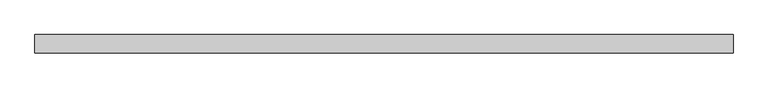
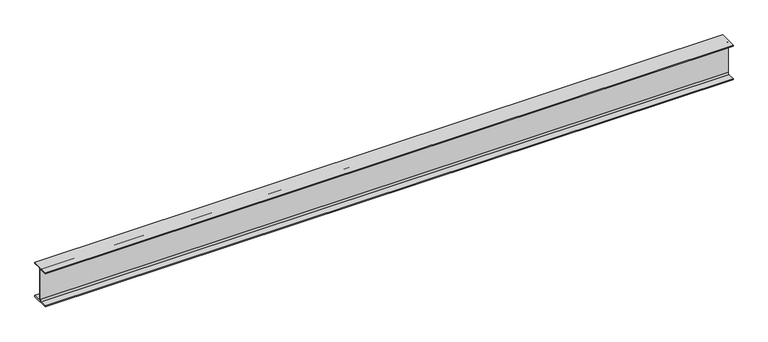
"""IFC4 building model written with IfcOpenShell, lengths in millimetres: beam geometry, Steel Framing_H_KS : H_SB_AR_S02_H-300x150x6.5x9_SRB3."""

from ifc_helpers import new_model, si_unit, point, frame, frame_2d, origin, place, context, project, spatial, polyline, circle_curve, trimmed, segment, composite_curve, outline, extrude, source, transform, mapped, element, save


def beam_c270cd18(model_context):
    return source(origin(), model_context, "Body", "SweptSolid", [
        extrude(outline(composite_curve([segment(polyline([(75.0, -141.0), (75.0, -150.0), (-75.0, -150.0), (-75.0, -141.0), (-16.25, -141.0)]), True, "CONTINUOUS"), segment(trimmed(circle_curve(frame_2d((-16.25, -128.0)), 13.0), [point((-16.25, -141.0))], [point((-3.25, -128.0))], True, "CARTESIAN"), True, "CONTINUOUS"), segment(polyline([(-3.25, -128.0), (-3.25, 128.0)]), True, "CONTINUOUS"), segment(trimmed(circle_curve(frame_2d((-16.25, 128.0)), 13.0), [point((-3.25, 128.0))], [point((-16.25, 141.0))], True, "CARTESIAN"), True, "CONTINUOUS"), segment(polyline([(-16.25, 141.0), (-75.0, 141.0), (-75.0, 150.0), (75.0, 150.0), (75.0, 141.0), (16.25, 141.0)]), True, "CONTINUOUS"), segment(trimmed(circle_curve(frame_2d((16.25, 128.0)), 13.0), [point((16.25, 141.0))], [point((3.25, 128.0))], True, "CARTESIAN"), True, "CONTINUOUS"), segment(polyline([(3.25, 128.0), (3.25, -128.0)]), True, "CONTINUOUS"), segment(trimmed(circle_curve(frame_2d((16.25, -128.0)), 13.0), [point((3.25, -128.0))], [point((16.25, -141.0))], True, "CARTESIAN"), True, "CONTINUOUS"), segment(polyline([(16.25, -141.0), (75.0, -141.0)]), True, "CONTINUOUS")], self_intersect=False)), frame((-2837.3, 0.0, 0.0), z_axis=(1.0, 0.0, 0.0), x_axis=(0.0, 1.0, 0.0)), (0.0, 0.0, 1.0), 5674.6),
    ])


if __name__ == "__main__":
    model = new_model("IFC4")
    model_context = context("Model", 3, world=origin())
    ifc_project = project(units=[si_unit("LENGTHUNIT", "METRE", prefix="MILLI")], contexts=[model_context])
    site = spatial("IfcSite", under=ifc_project)
    building = spatial("IfcBuilding", under=site)
    placement = place(None, origin())
    beam_shape = beam_c270cd18(model_context)
    element("IfcBeam", 1, ObjectType="Steel Framing_H_KS : H_SB_AR_S02_H-300x150x6.5x9_SRB3", at=placement, inside=building, context=model_context, shape_type="MappedRepresentation", body=[
        mapped(beam_shape, transform((0.0, 0.0, 0.0), x_axis=(1.0, 0.0, 0.0), y_axis=(0.0, 1.0, 0.0), z_axis=(0.0, 0.0, 1.0))),
    ])
    save(model, "model.ifc")

# Revit data of these elements
# Type "Steel Framing_H_KS : H_SB_AR_S02_H-300x150x6.5x9_SRB3"
#   Type Comments = "MAIN"
#   Type Mark = "SRB3"
#   H_SectionID = "H-300x150x6.5x9"
#   H_Ratio for Additional Steel Plate = 0.2
#   Width = 15.0 cm
#   Web Thickness = 0.65 cm
#   Web Fillet = 1.3 cm
#   Warping Constant = 107000.0 cm⁶
#   Torsional Moment of Inertia = 9.9539 cm⁴
#   Section Area = 46.78 cm²
#   Plastic Modulus weak axis = 105.0 cm³
#   Plastic Modulus strong axis = 542.0 cm³
#   Perimeter = 1.17 m²/m
#   Nominal Weight = 36.70 kgf/m
#   Moment of Inertia weak axis = 508.00 cm⁴
#   Moment of Inertia strong axis = 7210.00 cm⁴
#   Height = 30.0 cm
#   Flange Thickness = 0.9 cm
#   Elastic Modulus weak axis = 67.7 cm³
#   Elastic Modulus strong axis = 481.0 cm³
#   Centroid Vertical = 15.0 cm
#   Centroid Horizontal = 7.5 cm
#   Bolt Spacing = 8.89 cm
#   Length [instance default] = 1500 mm
#   Structural Material [instance default] = Steel, 45-345
#   Section Name Key = ""
#   Assembly Code = ""
# Element 1 (IfcBeam, "Steel Framing_H_KS : H_SB_AR_S02_H-300x150x6.5x9_SRB3")
#   Materials on its faces: "Steel, 45-345"
# Materials
#   "Steel, 45-345": class "Metal", colour RGB 189 187 185, transparency 0, Description = "Steel 345 MPa", Cost = 0
